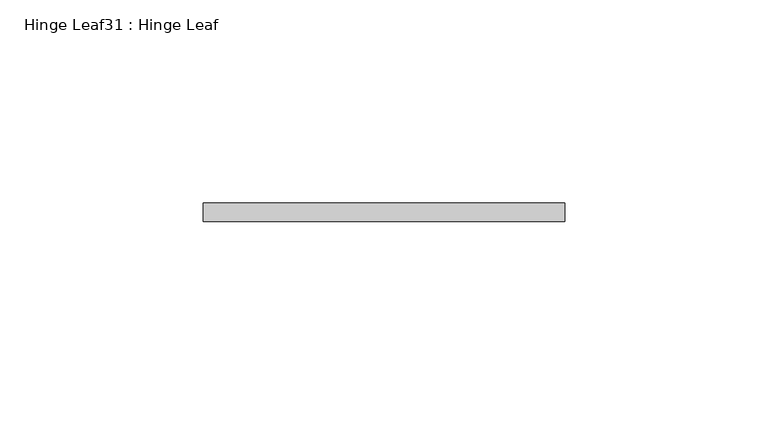
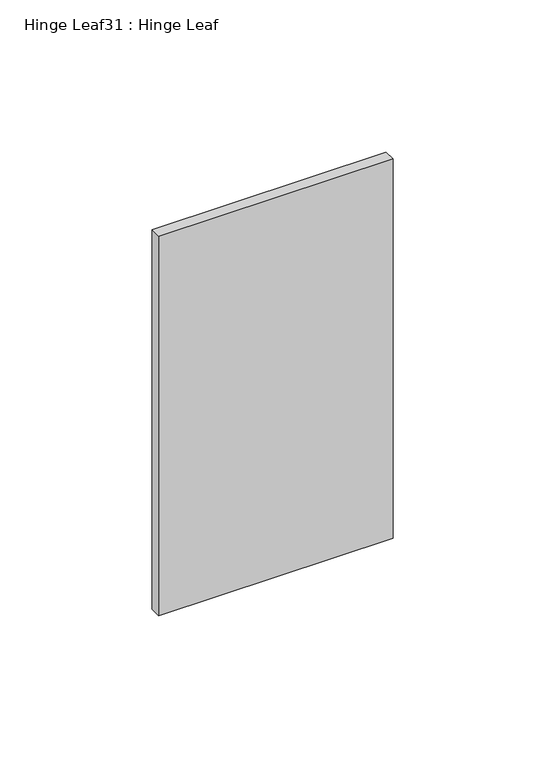
"""IFC4 building model written with IfcOpenShell, lengths in millimetres: proxy geometry, Hinge Leaf31 : Hinge Leaf."""

from ifc_helpers import new_model, si_unit, frame, origin, place, context, project, spatial, polyline, outline, extrude, source, transform, mapped, element, save


def hinge_leaf31_hinge_leaf_88ed8093(model_context):
    return source(origin(), model_context, "Body", "SweptSolid", [
        extrude(outline(polyline([(587327.7934739, -531772.5663841), (587416.6934739, -531772.5663841), (587416.6934739, -531777.1383841), (587327.7934739, -531777.1383841), (587327.7934739, -531772.5663841)])), frame((0.0, 0.0, 1123.95), z_axis=(0.0, 0.0, 1.0), x_axis=(1.0, 0.0, 0.0)), (0.0, 0.0, 1.0), 152.4),
    ])


if __name__ == "__main__":
    model = new_model("IFC4")
    model_context = context("Model", 3, world=origin())
    ifc_project = project(units=[si_unit("LENGTHUNIT", "METRE", prefix="MILLI")], contexts=[model_context])
    site = spatial("IfcSite", under=ifc_project)
    building = spatial("IfcBuilding", under=site)
    placement = place(None, origin())
    hinge_leaf31_hinge_leaf_shape = hinge_leaf31_hinge_leaf_88ed8093(model_context)
    element("IfcBuildingElementProxy", 1, Name="Hinge Leaf31 : Hinge Leaf", ObjectType="Hinge Leaf31 : Hinge Leaf", at=placement, inside=building, context=model_context, shape_type="MappedRepresentation", body=[
        mapped(hinge_leaf31_hinge_leaf_shape, transform((0.0, 0.0, 0.0), x_axis=(1.0, 0.0, 0.0), y_axis=(0.0, 1.0, 0.0), z_axis=(0.0, 0.0, 1.0))),
    ])
    save(model, "model.ifc")

# Revit data of these elements
# Element 1 (IfcBuildingElementProxy, "Hinge Leaf31 : Hinge Leaf")
#   Materials on its faces: "6\"X6\" WELD-ON STL BUTT HINGE"
# Materials
#   "6\"X6\" WELD-ON STL BUTT HINGE": class "Metal", colour RGB 189 187 185, transparency 0, Description = "Carbon steel", Cost = 0
